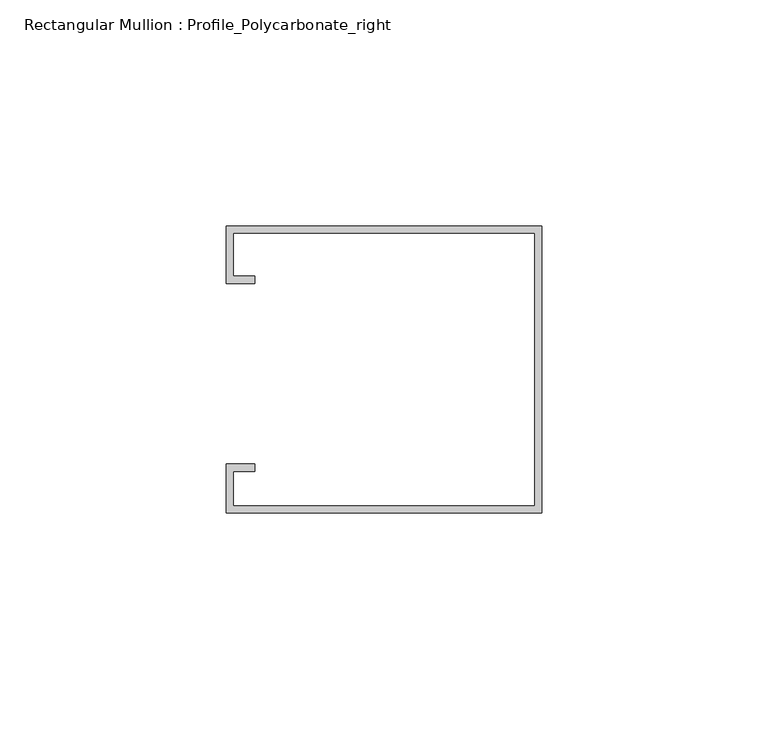
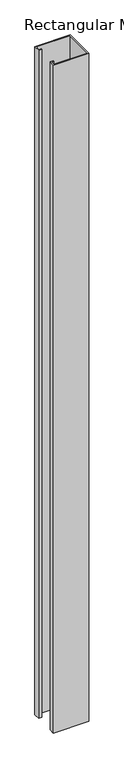
"""IFC4 building model written with IfcOpenShell, lengths in millimetres: member geometry, Rectangular Mullion : Profile_Polycarbonate_right."""

from ifc_helpers import new_model, si_unit, frame, origin, place, context, project, spatial, polyline, outline, extrude, source, transform, mapped, element, save


def rectangular_mullion_profile_polycarbonate_right_8b93aa93(model_context):
    return source(origin(), model_context, "Body", "SweptSolid", [
        extrude(outline(polyline([(0.0, 32.7), (0.0, -30.8), (-69.85, -30.8), (-69.85, -20.0), (-63.5, -20.0), (-63.5, -21.5875), (-68.2625, -21.5875), (-68.2625, -29.2125), (-1.5875, -29.2125), (-1.5875, 31.1125), (-68.2625, 31.1125), (-68.2625, 21.5875), (-63.5, 21.5875), (-63.5, 20.0), (-69.85, 20.0), (-69.85, 32.7), (0.0, 32.7)])), frame((0.0, 0.0, -1397.5422973), z_axis=(0.0, 0.0, 1.0), x_axis=(1.0, 0.0, 0.0)), (0.0, 0.0, 1.0), 1397.5422973),
    ])


if __name__ == "__main__":
    model = new_model("IFC4")
    model_context = context("Model", 3, world=origin())
    ifc_project = project(units=[si_unit("LENGTHUNIT", "METRE", prefix="MILLI")], contexts=[model_context])
    site = spatial("IfcSite", under=ifc_project)
    building = spatial("IfcBuilding", under=site)
    placement = place(None, origin())
    rectangular_mullion_profile_polycarbonate_right_shape = rectangular_mullion_profile_polycarbonate_right_8b93aa93(model_context)
    element("IfcMember", 1, ObjectType="Rectangular Mullion : Profile_Polycarbonate_right", at=placement, inside=building, context=model_context, shape_type="MappedRepresentation", body=[
        mapped(rectangular_mullion_profile_polycarbonate_right_shape, transform((0.0, 0.0, 0.0), x_axis=(1.0, 0.0, 0.0), y_axis=(0.0, 1.0, 0.0), z_axis=(0.0, 0.0, 1.0))),
    ])
    save(model, "model.ifc")

# Revit data of these elements
# Type "Rectangular Mullion : Profile_Polycarbonate_right"
#   built-in parameter 1007322 = 0.208333 (stored number, unit not read)
#   built-in parameter 1007321 = 0 (stored number, unit not read)
#   built-in parameter 1007320 = 0.00520833 (stored number, unit not read)
